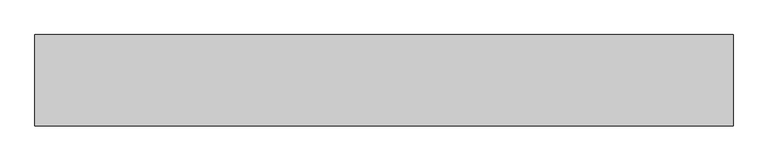
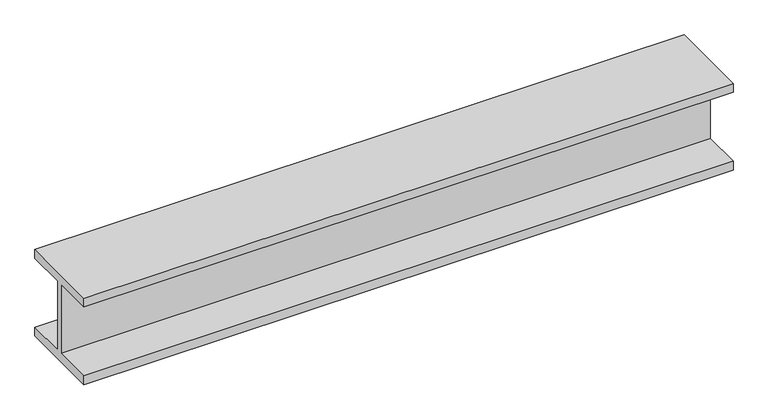
"""IFC4 building model written with IfcOpenShell, lengths in millimetres: proxy geometry, Structure054 5990 : Structure054 5990."""

import ifcopenshell
import ifcopenshell.guid

model = None  # the IFC model being written
_history = None  # IfcOwnerHistory: only IFC2X3 demands one
_inside = {}  # id of a spatial element -> (the spatial element, [elements in it])
_under = {}  # id of a project, library or spatial element -> (it, [spatial elements below it])
_declared = {}  # id of a project -> (the project, [libraries it declares])
_typed = {}  # id of a type object -> (the type object, [elements of that type])
_made_of = {}  # id of a material, layer set ... -> (it, [elements and type objects made of it])


def new_model(schema):
    """Start an empty IFC model of exactly this schema.

    Asked for "IFC4X3", IfcOpenShell would pick the latest addendum, in which some entities
    have other attributes; the version numbers below select the first issue.
    IFC2X3 requires an IfcOwnerHistory on every rooted entity: one is made here for all.
    """
    global model, _history
    if schema == "IFC4X3":
        model = ifcopenshell.file(schema_version=(4, 3, 0, 0))
    else:
        model = ifcopenshell.file(schema=schema)
    _inside.clear()
    _under.clear()
    _declared.clear()
    _typed.clear()
    _made_of.clear()
    _history = None
    if model.schema == "IFC2X3":
        org = make("IfcOrganization", Name="unknown")
        user = make(
            "IfcPersonAndOrganization",
            ThePerson=make("IfcPerson", FamilyName="unknown"),
            TheOrganization=org,
        )
        app = make(
            "IfcApplication",
            ApplicationDeveloper=org,
            Version="unknown",
            ApplicationFullName="unknown",
            ApplicationIdentifier="unknown",
        )
        _history = make(
            "IfcOwnerHistory",
            OwningUser=user,
            OwningApplication=app,
            ChangeAction="ADDED",
            CreationDate=0,
        )
    return model


def make(cls, **values):
    """One entity of the class cls with the attributes given. An attribute that is None is left unset."""
    return model.create_entity(
        cls, **{name: value for name, value in values.items() if value is not None}
    )


def rooted(cls, **values):
    """An entity with a GlobalId (a new one), such as an element, a storey or a relation."""
    return make(cls, GlobalId=ifcopenshell.guid.new(), OwnerHistory=_history, **values)


def si_unit(unit_type, name, prefix=None):
    """IfcSIUnit, for example si_unit("LENGTHUNIT", "METRE", prefix="MILLI")."""
    return make("IfcSIUnit", UnitType=unit_type, Prefix=prefix, Name=name)


def assignment(units):
    """IfcUnitAssignment: the units of a project."""
    return None if units is None else make("IfcUnitAssignment", Units=units)


def point(xyz):
    """IfcCartesianPoint."""
    return None if xyz is None else make("IfcCartesianPoint", Coordinates=xyz)


def direction(xyz):
    """IfcDirection."""
    return None if xyz is None else make("IfcDirection", DirectionRatios=xyz)


def frame(location, z_axis=None, x_axis=None):
    """IfcAxis2Placement3D, a coordinate frame: its origin and axes. An axis left out is left unset."""
    return make(
        "IfcAxis2Placement3D",
        Location=point(location),
        Axis=direction(z_axis),
        RefDirection=direction(x_axis),
    )


def origin():
    """The frame at (0, 0, 0) with its axes left unset."""
    return frame((0.0, 0.0, 0.0))


def place(relative_to, where):
    """IfcLocalPlacement: puts the frame where relative to a parent placement (None: the world)."""
    return make(
        "IfcLocalPlacement", PlacementRelTo=relative_to, RelativePlacement=where
    )


def context(
    kind, dimensions, precision=None, world=None, true_north=None, identifier=None
):
    """IfcGeometricRepresentationContext, for example the 3D "Model" context."""
    return make(
        "IfcGeometricRepresentationContext",
        ContextIdentifier=identifier,
        ContextType=kind,
        CoordinateSpaceDimension=dimensions,
        Precision=precision,
        WorldCoordinateSystem=world,
        TrueNorth=true_north,
    )


def project(units=None, contexts=None):
    """IfcProject with its units and contexts."""
    return rooted(
        "IfcProject",
        Name="project",
        RepresentationContexts=contexts,
        UnitsInContext=assignment(units),
    )


def spatial(cls, under=None, at=None, **own):
    """A site, building, storey or space (cls), placed at a placement, below another one or the project."""
    s = rooted(cls, ObjectPlacement=at, **own)
    if under is not None:
        _under.setdefault(under.id(), (under, []))[1].append(s)
    return s


def polyline(points):
    """IfcPolyline through the points."""
    return make("IfcPolyline", Points=[point(p) for p in points])


def outline(outer, holes=None, kind="AREA"):
    """IfcArbitraryClosedProfileDef: a profile drawn as a closed curve; with holes, ...WithVoids."""
    if holes is None:
        return make("IfcArbitraryClosedProfileDef", ProfileType=kind, OuterCurve=outer)
    return make(
        "IfcArbitraryProfileDefWithVoids",
        ProfileType=kind,
        OuterCurve=outer,
        InnerCurves=holes,
    )


def extrude(swept, where, along, depth):
    """IfcExtrudedAreaSolid: the profile swept, set in the frame where, extruded along a direction by depth."""
    return make(
        "IfcExtrudedAreaSolid",
        SweptArea=swept,
        Position=where,
        ExtrudedDirection=direction(along),
        Depth=depth,
    )


def shape(context_of_items, identifier, shape_type, items):
    """IfcShapeRepresentation: the items that make up one representation, for example the "Body"."""
    return make(
        "IfcShapeRepresentation",
        ContextOfItems=context_of_items,
        RepresentationIdentifier=identifier,
        RepresentationType=shape_type,
        Items=items,
    )


def source(mapping_origin, context_of_items, identifier, shape_type, items):
    """IfcRepresentationMap: a shape defined once, which mapped items show again and again."""
    return make(
        "IfcRepresentationMap",
        MappingOrigin=mapping_origin,
        MappedRepresentation=shape(context_of_items, identifier, shape_type, items),
    )


def transform(
    local_origin,
    x_axis=None,
    y_axis=None,
    z_axis=None,
    scale=None,
    scale2=None,
    scale3=None,
    uniform=True,
):
    """IfcCartesianTransformationOperator3D, or its non-uniform kind. x_axis, y_axis, z_axis: its Axis1, 2, 3."""
    if uniform:
        return make(
            "IfcCartesianTransformationOperator3D",
            Axis1=direction(x_axis),
            Axis2=direction(y_axis),
            LocalOrigin=point(local_origin),
            Scale=scale,
            Axis3=direction(z_axis),
        )
    return make(
        "IfcCartesianTransformationOperator3DnonUniform",
        Axis1=direction(x_axis),
        Axis2=direction(y_axis),
        LocalOrigin=point(local_origin),
        Scale=scale,
        Axis3=direction(z_axis),
        Scale2=scale2,
        Scale3=scale3,
    )


def mapped(mapping_source, mapping_target):
    """IfcMappedItem: shows the shape of a source again, moved by a transform."""
    return make(
        "IfcMappedItem", MappingSource=mapping_source, MappingTarget=mapping_target
    )


def made_of(thing, what):
    """Note that an element or type object is made of a material, layer set ...; save() writes the relation."""
    if what is not None:
        _made_of.setdefault(what.id(), (what, []))[1].append(thing)
    return thing


def element(
    cls,
    number,
    at=None,
    inside=None,
    cuts=None,
    type_object=None,
    material=None,
    context=None,
    identifier="Body",
    shape_type=None,
    held_by="IfcProductDefinitionShape",
    body=None,
    shapes=None,
    **own,
):
    """One element of the class cls, such as IfcWall. Its Tag is "e" and its number.

    at: its placement. inside: the storey or other place that contains it. cuts: it is an
    opening in that element (IfcRelVoidsElement). A single representation is given by context,
    identifier, shape_type and body (its items); several are given by shapes. held_by: the class
    of the entity that holds the representations. save() writes the other relations.
    """
    e = rooted(cls, Tag="e%d" % number, ObjectPlacement=at, **own)
    if body is not None:
        shapes = [shape(context, identifier, shape_type, body)]
    if shapes is not None:
        e.Representation = make(held_by, Representations=shapes)
    if inside is not None:
        _inside.setdefault(inside.id(), (inside, []))[1].append(e)
    if cuts is not None:
        rooted(
            "IfcRelVoidsElement", RelatingBuildingElement=cuts, RelatedOpeningElement=e
        )
    if type_object is not None:
        _typed.setdefault(type_object.id(), (type_object, []))[1].append(e)
    return made_of(e, material)


def aggregate(whole, parts):
    """IfcRelAggregates: a whole, such as a stair, and the parts it consists of."""
    return rooted("IfcRelAggregates", RelatingObject=whole, RelatedObjects=parts)


def save(model, path):
    """Write the relations noted so far, then the file.

    IfcRelAggregates (storeys below a building ...), IfcRelContainedInSpatialStructure (elements
    in a storey), IfcRelDefinesByType, IfcRelAssociatesMaterial and IfcRelDeclares: one each for
    every whole, place, type object, material and project.
    """
    for whole, parts in _under.values():
        aggregate(whole, parts)
    for where, things in _inside.values():
        rooted(
            "IfcRelContainedInSpatialStructure",
            RelatedElements=things,
            RelatingStructure=where,
        )
    for kind, things in _typed.values():
        rooted("IfcRelDefinesByType", RelatedObjects=things, RelatingType=kind)
    for what, things in _made_of.values():
        rooted("IfcRelAssociatesMaterial", RelatedObjects=things, RelatingMaterial=what)
    for by, libraries in _declared.values():
        rooted("IfcRelDeclares", RelatingContext=by, RelatedDefinitions=libraries)
    model.write(path)


def generic_models_b1736d61(model_context):
    return source(origin(), model_context, "Body", "SweptSolid", [
        extrude(outline(polyline([(-4211.4966368, 40049.1960937), (-4211.4966368, 40020.7480937), (-4333.668187, 40020.7480937), (-4333.668187, 39795.704), (-4211.4966368, 39795.704), (-4211.4966368, 39767.2560937), (-4473.1166368, 39767.2560937), (-4473.1166368, 39795.7040937), (-4350.940187, 39795.7040937), (-4350.940187, 40020.7480937), (-4473.1166368, 40020.7480937), (-4473.1166368, 40049.1960937), (-4211.4966368, 40049.1960937)])), frame((254.64, 0.0, 0.0), z_axis=(1.0, 0.0, 0.0), x_axis=(0.0, 1.0, 0.0)), (0.0, 0.0, 1.0), 2000.25),
    ])


if __name__ == "__main__":
    model = new_model("IFC4")
    model_context = context("Model", 3, world=origin())
    ifc_project = project(units=[si_unit("LENGTHUNIT", "METRE", prefix="MILLI")], contexts=[model_context])
    site = spatial("IfcSite", under=ifc_project)
    building = spatial("IfcBuilding", under=site)
    placement = place(None, origin())
    generic_models_shape = generic_models_b1736d61(model_context)
    element("IfcBuildingElementProxy", 1, Name="Structure054 5990 : Structure054 5990", ObjectType="Structure054 5990 : Structure054 5990", at=placement, inside=building, context=model_context, shape_type="MappedRepresentation", body=[
        mapped(generic_models_shape, transform((0.0, 0.0, 0.0), x_axis=(1.0, 0.0, 0.0), y_axis=(0.0, 1.0, 0.0), z_axis=(0.0, 0.0, 1.0))),
    ])
    save(model, "model.ifc")

# Revit data of these elements
# Type "Structure054 5990 : Structure054 5990"
#   NameOverride = "Structure054"
# Element 1 (IfcBuildingElementProxy, "Structure054 5990 : Structure054 5990")
#   Materials on its faces: "IfcSurfaceStyle #5964"
# Materials
#   "IfcSurfaceStyle #5964": class "Unassigned", colour RGB 150 169 186, transparency 0
